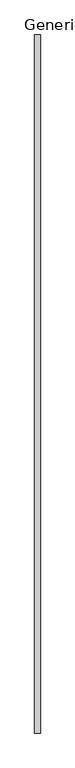
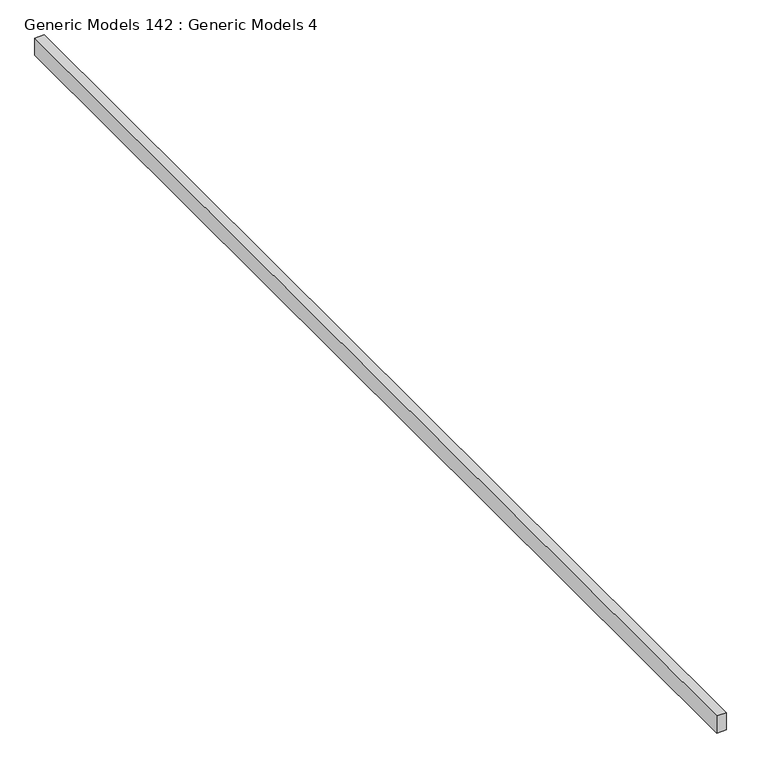
"""IFC4 building model written with IfcOpenShell, lengths in millimetres: proxy geometry, Generic Models 142 : Generic Models 4."""

from ifc_helpers import new_model, si_unit, frame, origin, place, context, project, spatial, polyline, outline, extrude, source, transform, mapped, element, save


def generic_models_142_generic_models_4_ea8f7fcb(model_context):
    return source(origin(), model_context, "Body", "SweptSolid", [
        extrude(outline(polyline([(-6629.5736296, -5493.3230338), (-6731.1736296, -5493.3230338), (-6731.1736296, 7054.2769662), (-6629.5736296, 7054.2769662), (-6629.5736296, -5493.3230338)])), frame((0.0, 0.0, 122955.6484874), z_axis=(0.0, 0.0, 1.0), x_axis=(1.0, 0.0, 0.0)), (0.0, 0.0, 1.0), 194.931421),
    ])


if __name__ == "__main__":
    model = new_model("IFC4")
    model_context = context("Model", 3, world=origin())
    ifc_project = project(units=[si_unit("LENGTHUNIT", "METRE", prefix="MILLI")], contexts=[model_context])
    site = spatial("IfcSite", under=ifc_project)
    building = spatial("IfcBuilding", under=site)
    placement = place(None, origin())
    generic_models_142_generic_models_4_shape = generic_models_142_generic_models_4_ea8f7fcb(model_context)
    element("IfcBuildingElementProxy", 1, Name="Generic Models 142 : Generic Models 4", ObjectType="Generic Models 142 : Generic Models 4", at=placement, inside=building, context=model_context, shape_type="MappedRepresentation", body=[
        mapped(generic_models_142_generic_models_4_shape, transform((0.0, 0.0, 0.0), x_axis=(1.0, 0.0, 0.0), y_axis=(0.0, 1.0, 0.0), z_axis=(0.0, 0.0, 1.0))),
    ])
    save(model, "model.ifc")

# Revit data of these elements
# Element 1 (IfcBuildingElementProxy, "Generic Models 142 : Generic Models 4")
#   Materials on its faces: "_LANDSCAPING STONE T.B.D."
# Materials
#   "_LANDSCAPING STONE T.B.D.": class "Generic", colour RGB 122 131 148, transparency 0, Cost = 0
